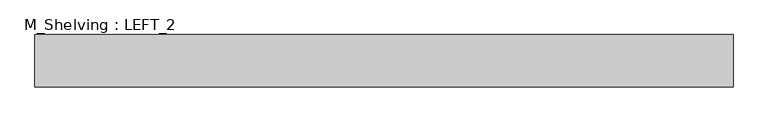
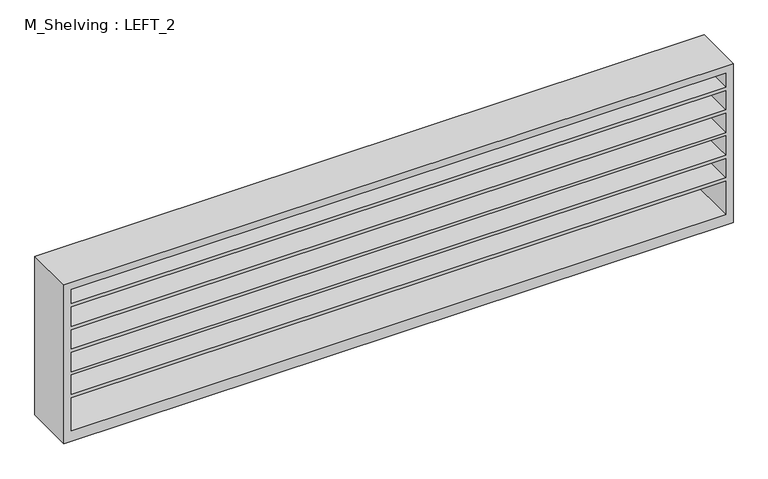
"""IFC4 building model written with IfcOpenShell, lengths in millimetres: furniture geometry, M_Shelving : LEFT_2."""

from ifc_helpers import new_model, si_unit, frame, origin, place, context, project, spatial, polyline, outline, extrude, source, transform, mapped, element, save


def m_shelving_left_2_f9164daf(model_context):
    return source(origin(), model_context, "Body", "SweptSolid", [
        extrude(outline(polyline([(0.0, 2330.0), (1170.0, 2330.0), (1170.0, -2330.0), (0.0, -2330.0), (0.0, 2330.0)]), holes=[polyline([(1119.2, 2279.2), (1015.5571429, 2279.2), (1015.5571429, -2279.2), (1119.2, -2279.2), (1119.2, 2279.2)]), polyline([(76.2, 2279.2), (76.2, -2279.2), (321.5857143, -2279.2), (321.5857143, 2279.2), (76.2, 2279.2)]), polyline([(681.2714286, -2279.2), (823.0142857, -2279.2), (823.0142857, 2279.2), (681.2714286, 2279.2), (681.2714286, -2279.2)]), polyline([(990.1571429, 2279.2), (848.4142857, 2279.2), (848.4142857, -2279.2), (990.1571429, -2279.2), (990.1571429, 2279.2)]), polyline([(655.8714286, 2279.2), (514.1285714, 2279.2), (514.1285714, -2279.2), (655.8714286, -2279.2), (655.8714286, 2279.2)]), polyline([(488.7285714, 2279.2), (346.9857143, 2279.2), (346.9857143, -2279.2), (488.7285714, -2279.2), (488.7285714, 2279.2)])]), frame((0.0, -479.8, 0.0), z_axis=(0.0, 1.0, 0.0), x_axis=(0.0, 0.0, 1.0)), (0.0, 0.0, 1.0), 350.0),
    ])


if __name__ == "__main__":
    model = new_model("IFC4")
    model_context = context("Model", 3, world=origin())
    ifc_project = project(units=[si_unit("LENGTHUNIT", "METRE", prefix="MILLI")], contexts=[model_context])
    site = spatial("IfcSite", under=ifc_project)
    building = spatial("IfcBuilding", under=site)
    placement = place(None, origin())
    m_shelving_left_2_shape = m_shelving_left_2_f9164daf(model_context)
    element("IfcFurniture", 1, ObjectType="M_Shelving : LEFT_2", at=placement, inside=building, context=model_context, shape_type="MappedRepresentation", body=[
        mapped(m_shelving_left_2_shape, transform((0.0, 0.0, 0.0), x_axis=(1.0, 0.0, 0.0), y_axis=(0.0, 1.0, 0.0), z_axis=(0.0, 0.0, 1.0))),
    ])
    save(model, "model.ifc")

# Revit data of these elements
# Type "M_Shelving : LEFT_2"
#   Depth = 350 mm
#   Height = 1170 mm
#   Width = 4660 mm
#   Material = Birch
#   Default Elevation = 0
# Element 1 (IfcFurniture, "M_Shelving : LEFT_2")
#   Materials on its faces: "Birch"
# Materials
#   "Birch": class "Wood", colour RGB 224 178 126, transparency 0, Description = "Betula Alleghaniensis", Cost = 0
